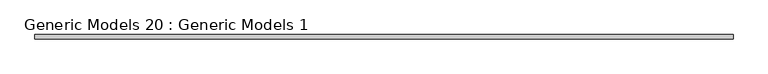
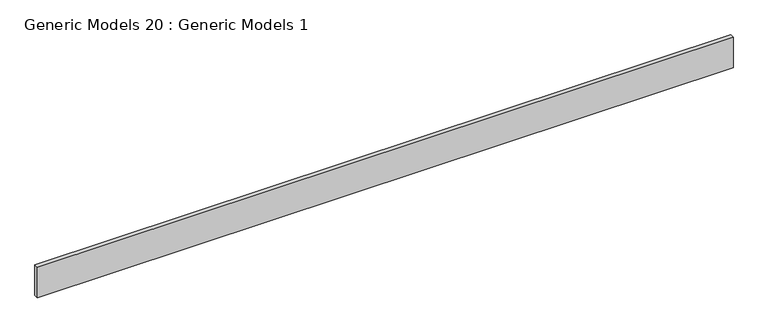
"""IFC4 building model written with IfcOpenShell, lengths in millimetres: proxy geometry, Generic Models 20 : Generic Models 1."""

from ifc_helpers import new_model, si_unit, frame, origin, place, context, project, spatial, polyline, outline, extrude, source, transform, mapped, element, save


def generic_models_20_generic_models_1_a654cbdf(model_context):
    return source(origin(), model_context, "Body", "SweptSolid", [
        extrude(outline(polyline([(2196.9263704, -7055.4230338), (2196.9263704, -7017.3230338), (8386.8578684, -7017.3230338), (8386.8578684, -7055.4230338), (2196.9263704, -7055.4230338)])), frame((0.0, 0.0, 126479.046), z_axis=(0.0, 0.0, 1.0), x_axis=(1.0, 0.0, 0.0)), (0.0, 0.0, 1.0), 285.75),
    ])


if __name__ == "__main__":
    model = new_model("IFC4")
    model_context = context("Model", 3, world=origin())
    ifc_project = project(units=[si_unit("LENGTHUNIT", "METRE", prefix="MILLI")], contexts=[model_context])
    site = spatial("IfcSite", under=ifc_project)
    building = spatial("IfcBuilding", under=site)
    placement = place(None, origin())
    generic_models_20_generic_models_1_shape = generic_models_20_generic_models_1_a654cbdf(model_context)
    element("IfcBuildingElementProxy", 1, Name="Generic Models 20 : Generic Models 1", ObjectType="Generic Models 20 : Generic Models 1", at=placement, inside=building, context=model_context, shape_type="MappedRepresentation", body=[
        mapped(generic_models_20_generic_models_1_shape, transform((0.0, 0.0, 0.0), x_axis=(1.0, 0.0, 0.0), y_axis=(0.0, 1.0, 0.0), z_axis=(0.0, 0.0, 1.0))),
    ])
    save(model, "model.ifc")

# Revit data of these elements
# Element 1 (IfcBuildingElementProxy, "Generic Models 20 : Generic Models 1")
#   Materials on its faces: "_STRUCTURAL MEMBER (SEE STRUCT. DWGS)"
# Materials
#   "_STRUCTURAL MEMBER (SEE STRUCT. DWGS)": class "Generic", colour RGB 209 182 141, transparency 0, Cost = 0
